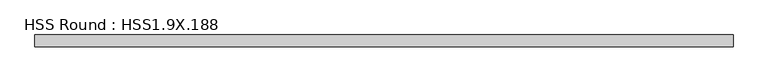
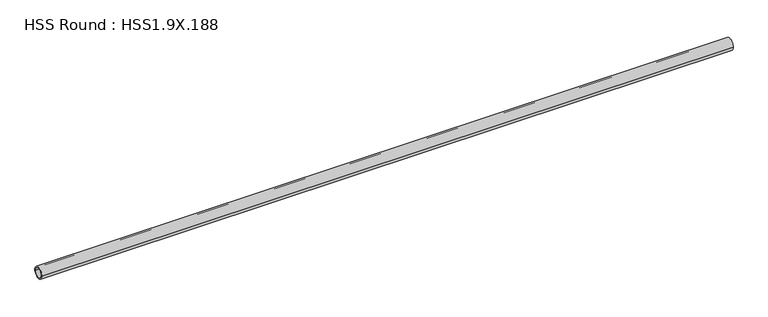
"""IFC4 building model written with IfcOpenShell, lengths in millimetres: member geometry, HSS Round : HSS1.9X.188."""

from ifc_helpers import new_model, si_unit, point, frame, origin, origin_2d, place, context, project, spatial, circle_curve, trimmed, segment, composite_curve, outline, extrude, source, transform, mapped, element, save


def hss_round_hss1_9x_188_ed40e31a(model_context):
    return source(origin(), model_context, "Body", "SweptSolid", [
        extrude(outline(composite_curve([segment(trimmed(circle_curve(origin_2d(), 24.13), [point((-24.13, 0.0))], [point((24.13, 0.0))], False, "CARTESIAN"), True, "CONTINUOUS"), segment(trimmed(circle_curve(origin_2d(), 24.13), [point((24.13, 0.0))], [point((-24.13, 0.0))], False, "CARTESIAN"), True, "CONTINUOUS")], self_intersect=False), holes=[composite_curve([segment(trimmed(circle_curve(origin_2d(), 19.3548), [point((19.3548, 0.0))], [point((-19.3548, 0.0))], True, "CARTESIAN"), True, "CONTINUOUS"), segment(trimmed(circle_curve(origin_2d(), 19.3548), [point((-19.3548, 0.0))], [point((19.3548, 0.0))], True, "CARTESIAN"), True, "CONTINUOUS")], self_intersect=False)]), frame((-1426.5365967, 0.0, 0.0), z_axis=(1.0, 0.0, 0.0), x_axis=(0.0, 1.0, 0.0)), (0.0, 0.0, 1.0), 2847.1284115),
    ])


if __name__ == "__main__":
    model = new_model("IFC4")
    model_context = context("Model", 3, world=origin())
    ifc_project = project(units=[si_unit("LENGTHUNIT", "METRE", prefix="MILLI")], contexts=[model_context])
    site = spatial("IfcSite", under=ifc_project)
    building = spatial("IfcBuilding", under=site)
    placement = place(None, origin())
    hss_round_hss1_9x_188_shape = hss_round_hss1_9x_188_ed40e31a(model_context)
    element("IfcMember", 1, ObjectType="HSS Round : HSS1.9X.188", at=placement, inside=building, context=model_context, shape_type="MappedRepresentation", body=[
        mapped(hss_round_hss1_9x_188_shape, transform((0.0, 0.0, 0.0), x_axis=(1.0, 0.0, 0.0), y_axis=(0.0, 1.0, 0.0), z_axis=(0.0, 0.0, 1.0))),
    ])
    save(model, "model.ifc")

# Revit data of these elements
# Type "HSS Round : HSS1.9X.188"
#   Section Name Key = "HSSRound 1.900x0.188"
#   Assembly Code = "B10"
#   Wall Nominal Thickness = 0.188"
#   Wall Design Thickness = 0.174"
#   Torsional Moment of Inertia = 0.71 in⁴
#   Torsional Modulus = 0.747 in³
#   Section Area = 0.943 in²
#   Plastic Modulus weak axis = 0.52 in³
#   Plastic Modulus strong axis = 0.52 in³
#   Nominal Weight = 3.44 lbf/ft
#   Moment of Inertia weak axis = 0.355 in⁴
#   Moment of Inertia strong axis = 0.355 in⁴
#   Elastic Modulus weak axis = 0.374 in³
#   Elastic Modulus strong axis = 0.374 in³
#   Diameter = 1.900"
#   Centroid Vertical = 0.950"
#   Centroid Horizontal = 0.950"
#   Length [instance default] = 5' - 0"
#   Structural Material [instance default] = Steel ASTM A500, Grade B, Round
#   Warping Constant = (empty or 0)
#   Principal Axes Angle = 0
# Element 1 (IfcMember, "HSS Round : HSS1.9X.188")
#   Structural Material = Steel ASTM A992
#   Materials on its faces: "Steel ASTM A992"
# Materials
#   "Steel ASTM A500, Grade B, Round": class "Metal", colour RGB 199 199 199, transparency 0, Description = "Carbon steel", Cost = 0
#   "Steel ASTM A992": class "Metal", colour RGB 199 199 199, transparency 0, Description = "Structural steel 50ksi", Cost = 0
